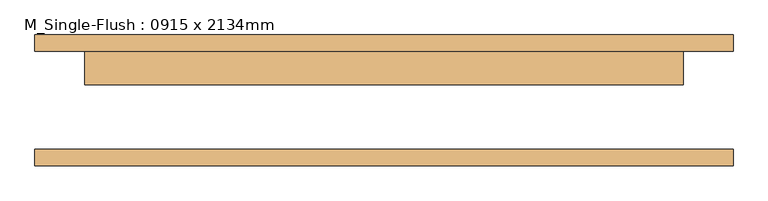
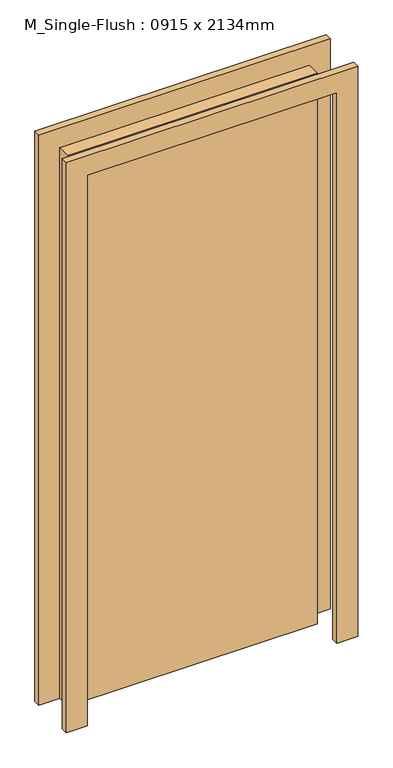
"""IFC4 building model written with IfcOpenShell, lengths in millimetres: door geometry, M_Single-Flush : 0915 x 2134mm."""

from ifc_helpers import new_model, si_unit, frame, origin, origin_with_axes, place, context, project, spatial, polyline, outline, extrude, source, transform, mapped, element, save


def m_single_flush_0915_x_2134mm_138fd904(model_context):
    return source(origin(), model_context, "Body", "SweptSolid", [
        extrude(outline(polyline([(2210.0, -533.5), (0.0, -533.5), (0.0, -457.5), (2134.0, -457.5), (2134.0, 457.5), (0.0, 457.5), (0.0, 533.5), (2210.0, 533.5), (2210.0, -533.5)])), frame((0.0, 75.0, 0.0), z_axis=(0.0, 1.0, 0.0), x_axis=(0.0, 0.0, 1.0)), (0.0, 0.0, 1.0), 25.0),
        extrude(outline(polyline([(2210.0, 533.5), (2210.0, -533.5), (0.0, -533.5), (0.0, -457.5), (2134.0, -457.5), (2134.0, 457.5), (0.0, 457.5), (0.0, 533.5), (2210.0, 533.5)])), frame((0.0, -100.0, 0.0), z_axis=(0.0, 1.0, 0.0), x_axis=(0.0, 0.0, 1.0)), (0.0, 0.0, 1.0), 25.0),
        extrude(outline(polyline([(457.5, 24.0), (-457.5, 24.0), (-457.5, 75.0), (457.5, 75.0), (457.5, 24.0)])), origin_with_axes(), (0.0, 0.0, 1.0), 2134.0),
    ])


if __name__ == "__main__":
    model = new_model("IFC4")
    model_context = context("Model", 3, world=origin())
    ifc_project = project(units=[si_unit("LENGTHUNIT", "METRE", prefix="MILLI")], contexts=[model_context])
    site = spatial("IfcSite", under=ifc_project)
    building = spatial("IfcBuilding", under=site)
    placement = place(None, origin())
    m_single_flush_0915_x_2134mm_shape = m_single_flush_0915_x_2134mm_138fd904(model_context)
    element("IfcDoor", 1, ObjectType="M_Single-Flush : 0915 x 2134mm", at=placement, inside=building, context=model_context, shape_type="MappedRepresentation", body=[
        mapped(m_single_flush_0915_x_2134mm_shape, transform((0.0, 0.0, 0.0), x_axis=(1.0, 0.0, 0.0), y_axis=(0.0, 1.0, 0.0), z_axis=(0.0, 0.0, 1.0))),
    ])
    save(model, "model.ifc")

# Revit data of these elements
# Type "M_Single-Flush : 0915 x 2134mm"
#   Type Mark = "15"
#   Thickness = 0.051 m
#   Height = 2.134 m
#   Trim Projection Ext = 0.025 m
#   Trim Projection Int = 0.025 m
#   Trim Width = 0.076 m
#   Width = 0.915 m
#   Door Material = Door - Panel
#   Frame Material = Door - Frame
#   Function = (empty or 0)
#   Wall Closure = (empty or 0)
# Element 1 (IfcDoor, "M_Single-Flush : 0915 x 2134mm")
#   Materials on its faces: "Door - Frame", "Door - Panel"
# Materials
#   "Door - Panel": class "Wood", colour RGB 114 82 51, transparency 0
#   "Door - Frame": class "Miscellaneous", colour RGB 255 0 128, transparency 0, Cost = 0
